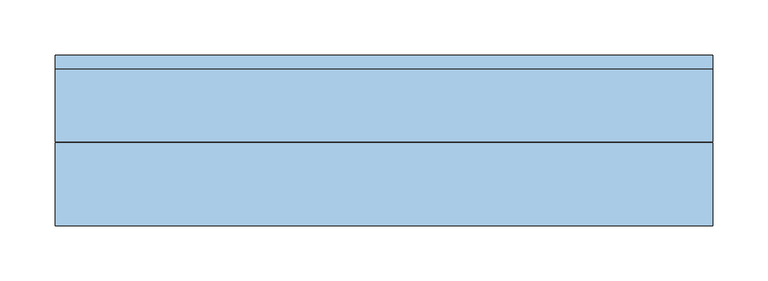
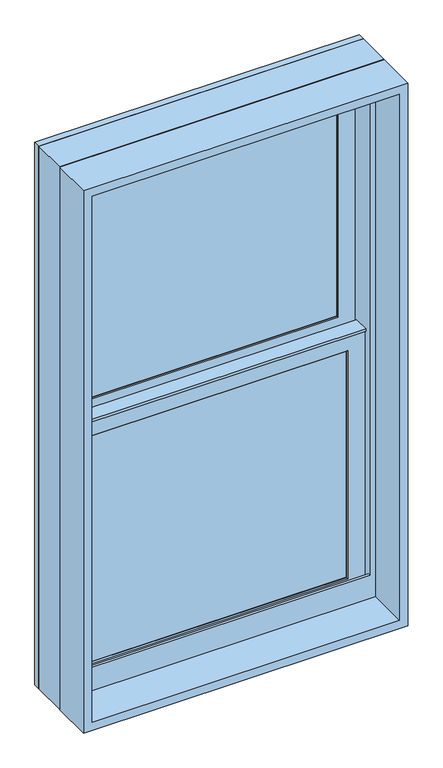
"""IFC4 building model written with IfcOpenShell, lengths in millimetres: window geometry, Window-Double_Hung-Marvin-Essential : ESDH2036."""

from ifc_helpers import new_model, si_unit, frame, origin, place, context, project, spatial, polyline, outline, extrude, faceted_brep, source, transform, mapped, element, save


def window_21fe58db(model_context):
    return source(origin(), model_context, "Body", "SolidModel", [
        extrude(outline(polyline([(89.9583333, 20.6375), (89.9583333, 15.875), (70.9083333, 15.875), (70.9083333, 20.6375), (89.9583333, 20.6375)])), frame((0.0, 0.0, 1441.45), z_axis=(0.0, 0.0, 1.0), x_axis=(1.0, 0.0, 0.0)), (0.0, 0.0, 1.0), 450.85),
        extrude(outline(polyline([(-70.9083333, 20.6375), (-70.9083333, 15.875), (-89.9583333, 15.875), (-89.9583333, 20.6375), (-70.9083333, 20.6375)])), frame((0.0, 0.0, 1441.45), z_axis=(0.0, 0.0, 1.0), x_axis=(1.0, 0.0, 0.0)), (0.0, 0.0, 1.0), 450.85),
        extrude(outline(polyline([(241.3, 20.6375), (241.3, 15.875), (-241.3, 15.875), (-241.3, 20.6375), (241.3, 20.6375)])), frame((0.0, 0.0, 1657.35), z_axis=(0.0, 0.0, 1.0), x_axis=(1.0, 0.0, 0.0)), (0.0, 0.0, 1.0), 19.05),
        extrude(outline(polyline([(-89.9583333, 46.83125), (-89.9583333, 51.59375), (-70.9083333, 51.59375), (-70.9083333, 46.83125), (-89.9583333, 46.83125)])), frame((0.0, 0.0, 1930.4), z_axis=(0.0, 0.0, 1.0), x_axis=(1.0, 0.0, 0.0)), (0.0, 0.0, 1.0), 450.85),
        extrude(outline(polyline([(70.9083333, 46.83125), (70.9083333, 51.59375), (89.9583333, 51.59375), (89.9583333, 46.83125), (70.9083333, 46.83125)])), frame((0.0, 0.0, 1930.4), z_axis=(0.0, 0.0, 1.0), x_axis=(1.0, 0.0, 0.0)), (0.0, 0.0, 1.0), 450.85),
        extrude(outline(polyline([(-241.3, 46.83125), (-241.3, 51.59375), (241.3, 51.59375), (241.3, 46.83125), (-241.3, 46.83125)])), frame((0.0, 0.0, 2146.3), z_axis=(0.0, 0.0, 1.0), x_axis=(1.0, 0.0, 0.0)), (0.0, 0.0, 1.0), 19.05),
        extrude(outline(polyline([(89.9583333, 20.6375), (70.9083333, 20.6375), (70.9083333, 25.4), (89.9583333, 25.4), (89.9583333, 20.6375)])), frame((0.0, 0.0, 1441.45), z_axis=(0.0, 0.0, 1.0), x_axis=(1.0, 0.0, 0.0)), (0.0, 0.0, 1.0), 450.85),
        extrude(outline(polyline([(-70.9083333, 20.6375), (-89.9583333, 20.6375), (-89.9583333, 25.4), (-70.9083333, 25.4), (-70.9083333, 20.6375)])), frame((0.0, 0.0, 1441.45), z_axis=(0.0, 0.0, 1.0), x_axis=(1.0, 0.0, 0.0)), (0.0, 0.0, 1.0), 450.85),
        extrude(outline(polyline([(241.3, 20.6375), (-241.3, 20.6375), (-241.3, 25.4), (241.3, 25.4), (241.3, 20.6375)])), frame((0.0, 0.0, 1657.35), z_axis=(0.0, 0.0, 1.0), x_axis=(1.0, 0.0, 0.0)), (0.0, 0.0, 1.0), 19.05),
        extrude(outline(polyline([(-89.9583333, 56.35625), (-70.9083333, 56.35625), (-70.9083333, 51.59375), (-89.9583333, 51.59375), (-89.9583333, 56.35625)])), frame((0.0, 0.0, 1930.4), z_axis=(0.0, 0.0, 1.0), x_axis=(1.0, 0.0, 0.0)), (0.0, 0.0, 1.0), 450.85),
        extrude(outline(polyline([(70.9083333, 56.35625), (89.9583333, 56.35625), (89.9583333, 51.59375), (70.9083333, 51.59375), (70.9083333, 56.35625)])), frame((0.0, 0.0, 1930.4), z_axis=(0.0, 0.0, 1.0), x_axis=(1.0, 0.0, 0.0)), (0.0, 0.0, 1.0), 450.85),
        extrude(outline(polyline([(-241.3, 56.35625), (241.3, 56.35625), (241.3, 51.59375), (-241.3, 51.59375), (-241.3, 56.35625)])), frame((0.0, 0.0, 2146.3), z_axis=(0.0, 0.0, 1.0), x_axis=(1.0, 0.0, 0.0)), (0.0, 0.0, 1.0), 19.05),
        faceted_brep([(-268.2875, 5.6780605, 1922.3351748), (-268.2875, 5.6780605, 1917.7), (268.2875, 5.6780605, 1917.7), (268.2875, 5.6780605, 1922.3351748), (-268.2875, 34.8118605, 1922.3351748), (268.2875, 34.8118605, 1922.3351748), (268.2875, 34.8118605, 1917.7), (-268.2875, 34.8118605, 1917.7), (-268.2875, 30.1625, 1917.7), (-268.2875, 30.1625, 1414.4625), (-268.2875, 8.9241104, 1414.4625), (-268.2875, 8.9241104, 1917.7), (268.2875, 8.9241104, 1917.7), (268.2875, 30.1625, 1917.7), (268.2875, 8.9241104, 1414.4625), (268.2875, 30.1625, 1414.4625), (-252.4034752, 11.90625, 1903.4034752), (-252.4034752, 30.1625, 1903.4034752), (252.4034752, 30.1625, 1903.4034752), (252.4034752, 11.90625, 1903.4034752), (-235.74375, 10.4662439, 1886.74375), (-235.74375, 11.90625, 1886.74375), (235.74375, 11.90625, 1886.74375), (235.74375, 10.4662439, 1886.74375), (237.2858834, 8.9241104, 1888.2858834), (-237.2858834, 8.9241104, 1888.2858834), (252.4034752, 30.1625, 1430.3465248), (252.4034752, 11.90625, 1430.3465248), (235.74375, 11.90625, 1447.00625), (235.74375, 10.4662439, 1447.00625), (237.2858834, 8.9241104, 1445.4641166), (-252.4034752, 30.1625, 1430.3465248), (-252.4034752, 11.90625, 1430.3465248), (-235.74375, 11.90625, 1447.00625), (-235.74375, 10.4662439, 1447.00625), (-237.2858834, 8.9241104, 1445.4641166)], [[[0, 1, 2, 3]], [[4, 5, 6, 7]], [[1, 0, 4, 7, 8, 9, 10, 11]], [[2, 1, 11, 12]], [[7, 6, 13, 8]], [[3, 2, 12, 14, 15, 13, 6, 5]], [[0, 3, 5, 4]], [[16, 17, 18, 19]], [[20, 21, 22, 23]], [[20, 23, 24, 25]], [[19, 18, 26, 27]], [[23, 22, 28, 29]], [[24, 23, 29, 30]], [[27, 26, 31, 32]], [[29, 28, 33, 34]], [[30, 29, 34, 35]], [[15, 14, 10, 9]], [[15, 9, 8, 13], [18, 17, 31, 26]], [[17, 16, 32, 31]], [[16, 19, 27, 32], [22, 21, 33, 28]], [[21, 20, 34, 33]], [[20, 25, 35, 34]], [[10, 14, 12, 11], [25, 24, 30, 35]]]),
        extrude(outline(polyline([(38.5955581, 1903.4125), (33.5778968, 1903.4125), (33.5778968, 1905.0), (39.9405976, 1905.0), (39.9405976, 1903.4125), (61.515625, 1903.4125), (47.6307501, 1900.0975159), (38.5955581, 1900.0975159), (38.5955581, 1903.4125)])), frame((-268.2875, 0.0, 0.0), z_axis=(1.0, 0.0, 0.0), x_axis=(0.0, 1.0, 0.0)), (0.0, 0.0, 1.0), 536.575),
        faceted_brep([(298.45, 0.0, 1384.3), (298.45, 0.0, 2438.4), (-298.45, 0.0, 2438.4), (-298.45, 0.0, 1384.3), (272.25625, 0.0, 1445.41875), (-272.25625, 0.0, 1445.41875), (-272.25625, 0.0, 2412.20625), (272.25625, 0.0, 2412.20625), (272.25625, 3.96875, 1384.3), (-272.25625, 3.96875, 1384.3), (-272.25625, 3.96875, 1445.41875), (272.25625, 3.96875, 1445.41875), (-298.45, 65.6828125, 1384.3), (-272.25625, 65.6828125, 1384.3), (272.25625, 65.6828125, 1384.3), (298.45, 65.6828125, 1384.3), (-298.45, 65.6828125, 2438.4), (298.45, 65.6828125, 2438.4), (272.25625, 65.6828125, 2412.20625), (-272.25625, 65.6828125, 2412.20625)], [[[0, 1, 2, 3], [4, 5, 6, 7]], [[8, 9, 10, 11]], [[5, 4, 11, 10]], [[0, 3, 12, 13, 9, 8, 14, 15]], [[13, 12, 16, 17, 15, 14, 18, 19]], [[13, 19, 6, 5, 10, 9]], [[7, 6, 19, 18]], [[18, 14, 8, 11, 4, 7]], [[1, 0, 15, 17]], [[2, 1, 17, 16]], [[3, 2, 16, 12]]]),
        faceted_brep([(272.25625, 30.1625, 1911.35), (270.66875, 30.1625, 1911.35), (270.66875, 30.1625, 1408.6544613), (272.25625, 30.1625, 1408.6544613), (-270.66875, 30.1625, 1911.35), (-272.25625, 30.1625, 1911.35), (-272.25625, 30.1625, 1408.6544613), (-270.66875, 30.1625, 1408.6544613), (270.66875, 63.5, 1911.35), (272.25625, 63.5, 1911.35), (272.25625, 63.5, 1402.1743077), (270.66875, 63.5, 1402.1743077), (-272.25625, 63.5, 1911.35), (-270.66875, 63.5, 1911.35), (-270.66875, 63.5, 1402.1743077), (-272.25625, 63.5, 1402.1743077), (283.5108932, 3.96875, 1413.7460105), (283.5108932, 3.96875, 1384.3), (283.5108932, 65.6828125, 1384.3), (283.5108932, 65.6828125, 1401.750012), (-283.5108932, 3.96875, 1384.3), (-283.5108932, 3.96875, 1413.7460105), (-283.5108932, 65.6828125, 1401.750012), (-283.5108932, 65.6828125, 1384.3), (283.5108932, 78.58125, 1399.2428097), (-283.5108932, 78.58125, 1399.2428097), (-281.4971252, 68.2348864, 1401.2539391), (-263.53135, 68.2348864, 1401.2539391), (-263.53135, 65.6828125, 1401.750012), (263.53135, 65.6828125, 1401.750012), (263.53135, 68.2348864, 1401.2539391), (281.4971252, 68.2348864, 1401.2539391), (-298.45, 65.6828125, 1384.3), (-298.45, 78.5948249, 1384.3), (298.45, 78.5948249, 1384.3), (298.45, 65.6828125, 1384.3), (-298.45, 78.58125, 2438.4), (298.45, 78.58125, 2438.4), (283.5108932, 78.58125, 2423.4608932), (-283.5108932, 78.58125, 2423.4608932), (-298.45, 65.6828125, 2438.4), (-281.4971252, 68.2348864, 2421.4471252), (281.4971252, 68.2348864, 2421.4471252), (263.53135, 68.2348864, 2403.48135), (-263.53135, 68.2348864, 2403.48135), (-263.53135, 65.6828125, 2403.48135), (263.53135, 65.6828125, 2403.48135), (298.45, 65.6828125, 2438.4)], [[[0, 1, 2, 3]], [[4, 5, 6, 7]], [[8, 9, 10, 11]], [[12, 13, 14, 15]], [[1, 8, 11, 2]], [[9, 0, 3, 10]], [[1, 0, 9, 8]], [[5, 4, 13, 12]], [[5, 12, 15, 6]], [[13, 4, 7, 14]], [[16, 17, 18, 19]], [[20, 21, 22, 23]], [[24, 25, 26, 27, 28, 22, 21, 16, 19, 29, 30, 31], [3, 2, 11, 10], [7, 6, 15, 14]], [[17, 16, 21, 20]], [[17, 20, 23, 32, 33, 34, 35, 18]], [[34, 33, 36, 37], [25, 24, 38, 39]], [[33, 32, 40, 36]], [[39, 41, 26, 25]], [[41, 42, 31, 30, 43, 44, 27, 26]], [[44, 45, 28, 27]], [[40, 32, 23, 22, 28, 45, 46, 29, 19, 18, 35, 47]], [[36, 40, 47, 37]], [[39, 38, 42, 41]], [[44, 43, 46, 45]], [[34, 37, 47, 35]], [[42, 38, 24, 31]], [[46, 43, 30, 29]]]),
        extrude(outline(polyline([(248.44375, 11.90625), (-248.44375, 11.90625), (-248.44375, 15.08125), (248.44375, 15.08125), (248.44375, 11.90625)])), frame((0.0, 0.0, 1434.30625), z_axis=(0.0, 0.0, 1.0), x_axis=(1.0, 0.0, 0.0)), (0.0, 0.0, 1.0), 465.1375),
        extrude(outline(polyline([(248.44375, 42.8625), (-248.44375, 42.8625), (-248.44375, 46.0375), (248.44375, 46.0375), (248.44375, 42.8625)])), frame((0.0, 0.0, 1923.25625), z_axis=(0.0, 0.0, 1.0), x_axis=(1.0, 0.0, 0.0)), (0.0, 0.0, 1.0), 465.1375),
        faceted_brep([(-235.74375, 31.194477, 1886.74375), (-237.2858834, 32.7366104, 1888.2858834), (237.2858834, 32.7366104, 1888.2858834), (235.74375, 31.194477, 1886.74375), (-235.74375, 30.1625, 1886.74375), (235.74375, 30.1625, 1886.74375), (-268.2875, 32.7366104, 1919.2875), (-268.2875, 30.1625, 1919.2875), (268.2875, 30.1625, 1919.2875), (268.2875, 32.7366104, 1919.2875), (237.2858834, 32.7366104, 1445.4641166), (235.74375, 31.194477, 1447.00625), (235.74375, 30.1625, 1447.00625), (268.2875, 30.1625, 1414.4625), (268.2875, 32.7366104, 1414.4625), (-237.2858834, 32.7366104, 1445.4641166), (-235.74375, 31.194477, 1447.00625), (-235.74375, 30.1625, 1447.00625), (-268.2875, 30.1625, 1414.4625), (-268.2875, 32.7366104, 1414.4625)], [[[0, 1, 2, 3]], [[4, 0, 3, 5]], [[6, 7, 8, 9]], [[3, 2, 10, 11]], [[5, 3, 11, 12]], [[9, 8, 13, 14]], [[11, 10, 15, 16]], [[12, 11, 16, 17]], [[14, 13, 18, 19]], [[9, 14, 19, 6], [1, 15, 10, 2]], [[16, 15, 1, 0]], [[17, 16, 0, 4]], [[7, 18, 13, 8], [5, 12, 17, 4]], [[19, 18, 7, 6]]]),
        faceted_brep([(-252.4034752, 42.8625, 2392.3534752), (-252.4034752, 61.11875, 2392.3534752), (252.4034752, 61.11875, 2392.3534752), (252.4034752, 42.8625, 2392.3534752), (-235.74375, 41.4224939, 2375.69375), (-235.74375, 42.8625, 2375.69375), (235.74375, 42.8625, 2375.69375), (235.74375, 41.4224939, 2375.69375), (-237.2858834, 39.8803604, 2377.2358834), (237.2858834, 39.8803604, 2377.2358834), (-268.2875, 61.11875, 2408.2375), (-268.2875, 39.8803604, 2408.2375), (268.2875, 39.8803604, 2408.2375), (268.2875, 61.11875, 2408.2375), (252.4034752, 61.11875, 1919.2965248), (252.4034752, 42.8625, 1919.2965248), (235.74375, 42.8625, 1935.95625), (235.74375, 41.4224939, 1935.95625), (237.2858834, 39.8803604, 1934.4141166), (268.2875, 39.8803604, 1903.4125), (268.2875, 61.11875, 1903.4125), (-252.4034752, 61.11875, 1919.2965248), (-252.4034752, 42.8625, 1919.2965248), (-235.74375, 42.8625, 1935.95625), (-235.74375, 41.4224939, 1935.95625), (-237.2858834, 39.8803604, 1934.4141166), (-268.2875, 39.8803604, 1903.4125), (-268.2875, 61.11875, 1903.4125)], [[[0, 1, 2, 3]], [[4, 5, 6, 7]], [[8, 4, 7, 9]], [[10, 11, 12, 13]], [[3, 2, 14, 15]], [[7, 6, 16, 17]], [[9, 7, 17, 18]], [[13, 12, 19, 20]], [[15, 14, 21, 22]], [[17, 16, 23, 24]], [[18, 17, 24, 25]], [[20, 19, 26, 27]], [[13, 20, 27, 10], [1, 21, 14, 2]], [[22, 21, 1, 0]], [[3, 15, 22, 0], [5, 23, 16, 6]], [[24, 23, 5, 4]], [[25, 24, 4, 8]], [[11, 26, 19, 12], [9, 18, 25, 8]], [[27, 26, 11, 10]]]),
        faceted_brep([(-268.2875, 61.11875, 1903.4125), (-268.2875, 63.6928604, 1903.4125), (268.2875, 63.6928604, 1903.4125), (268.2875, 61.11875, 1903.4125), (-235.74375, 62.150727, 1935.95625), (-235.74375, 61.11875, 1935.95625), (235.74375, 61.11875, 1935.95625), (235.74375, 62.150727, 1935.95625), (-237.2858834, 63.6928604, 1934.4141166), (237.2858834, 63.6928604, 1934.4141166), (268.2875, 63.6928604, 2408.2375), (268.2875, 61.11875, 2408.2375), (235.74375, 61.11875, 2375.69375), (235.74375, 62.150727, 2375.69375), (237.2858834, 63.6928604, 2377.2358834), (-268.2875, 63.6928604, 2408.2375), (-268.2875, 61.11875, 2408.2375), (-235.74375, 61.11875, 2375.69375), (-235.74375, 62.150727, 2375.69375), (-237.2858834, 63.6928604, 2377.2358834)], [[[0, 1, 2, 3]], [[4, 5, 6, 7]], [[8, 4, 7, 9]], [[3, 2, 10, 11]], [[7, 6, 12, 13]], [[9, 7, 13, 14]], [[11, 10, 15, 16]], [[13, 12, 17, 18]], [[14, 13, 18, 19]], [[16, 15, 1, 0]], [[3, 11, 16, 0], [5, 17, 12, 6]], [[18, 17, 5, 4]], [[19, 18, 4, 8]], [[1, 15, 10, 2], [9, 14, 19, 8]]]),
        extrude(outline(polyline([(248.44375, 26.19375), (-248.44375, 26.19375), (-248.44375, 30.1625), (248.44375, 30.1625), (248.44375, 26.19375)])), frame((0.0, 0.0, 1434.30625), z_axis=(0.0, 0.0, 1.0), x_axis=(1.0, 0.0, 0.0)), (0.0, 0.0, 1.0), 465.1375),
        extrude(outline(polyline([(248.44375, 57.15), (-248.44375, 57.15), (-248.44375, 61.11875), (248.44375, 61.11875), (248.44375, 57.15)])), frame((0.0, 0.0, 1923.25625), z_axis=(0.0, 0.0, 1.0), x_axis=(1.0, 0.0, 0.0)), (0.0, 0.0, 1.0), 465.1375),
        extrude(outline(polyline([(2438.4, 298.45), (2438.4, -298.45), (1384.3, -298.45), (1384.3, 298.45), (2438.4, 298.45)]), holes=[polyline([(2422.525, 282.575), (1400.175, 282.575), (1400.175, -282.575), (2422.525, -282.575), (2422.525, 282.575)])]), frame((0.0, -76.2, 0.0), z_axis=(0.0, 1.0, 0.0), x_axis=(0.0, 0.0, 1.0)), (0.0, 0.0, 1.0), 75.40625),
    ])


if __name__ == "__main__":
    model = new_model("IFC4")
    model_context = context("Model", 3, world=origin())
    ifc_project = project(units=[si_unit("LENGTHUNIT", "METRE", prefix="MILLI")], contexts=[model_context])
    site = spatial("IfcSite", under=ifc_project)
    building = spatial("IfcBuilding", under=site)
    placement = place(None, origin())
    window_shape = window_21fe58db(model_context)
    element("IfcWindow", 1, ObjectType="Window-Double_Hung-Marvin-Essential : ESDH2036", at=placement, inside=building, context=model_context, shape_type="MappedRepresentation", body=[
        mapped(window_shape, transform((0.0, 0.0, 0.0), x_axis=(1.0, 0.0, 0.0), y_axis=(0.0, 1.0, 0.0), z_axis=(0.0, 0.0, 1.0))),
    ])
    save(model, "model.ifc")

# Revit data of these elements
# Type "Window-Double_Hung-Marvin-Essential : ESDH2036"
#   Type Mark = "41"
#   Window Type = "Essential Double Hung"
#   Product data url = "https://bimobject.com/marvin-windows-and-doors/product/marvin-dhwau"
#   Product Guid = "c4a96547-874c-4385-91dc-a058adc19d98"
#   Frame = "All Ultrex"
#   Egress Window = "No"
#   URL = "www.marvin.com"
#   Model = "ESDH2036"
#   Manufacturer = "Marvin Windows and Doors"
#   Label Egress = ""
#   Glass Type = "IG Low E II with Argon"
#   Design Pressure = "DP50"
#   Description = "2442 DBHG"
#   Analytic Construction = "<None>"
#   Prairie Corner Width = 0' - 4"
#   Prairie Corner Height = 0' - 4"
#   Egress Width = 1' - 8 9/16"
#   Egress Height = 1' - 4 27/128"
#   Rough Width = 2' - 0"
#   Rough Height = 3' - 6"
#   Nominal Width = 2' - 0"
#   Nominal Height = 3' - 6"
#   Inset to Installation Flange [instance default] = 0' - 1"
#   Height = 3' - 5 1/2"
#   Egress Area = 2.31484 SF
#   Default Head Height = 8' - 0"
#   Width = 1' - 11 1/2"
#   Daylight Area = 4.46338 SF
#   DLO Width = 1' - 6 9/16"
#   DLO Height = 1' - 5 5/16"
#   Muntins Top Sash = yes
#   Lites Wide Top Sash = 3
#   Lites Wide Bottom Sash = 3
#   Lites High Top Sash = 2
#   Lites High Bottom Sash = 2
#   Lite Cut Prairie 9 = no
#   Lite Cut HV Grid = yes
#   Muntins Bottom Sash = yes
#   Label Visibility = no
#   Jamb Extension Visibility = yes
#   Edition number = 1
#   Interior Material = Ultrex-Marvin-Stonewhite
#   Glazing Material = Glass-Marvin-IG Low E II with Argon
#   Cladding Material = Ultrex-Marvin-Pebblegray
#   Wall Closure = (empty or 0)
#   Assembly Code = ""
# Element 1 (IfcWindow, "Window-Double_Hung-Marvin-Essential : ESDH2036")
#   Materials on its faces: "Ultrex-Marvin-Pebblegray", "Ultrex-Marvin-Stonewhite", "Glass-Marvin-IG Low E II with Argon"
# Materials
#   "Ultrex-Marvin-Stonewhite": class "Paint", colour RGB 250 251 245, transparency 0
#   "Glass-Marvin-IG Low E II with Argon": class "Glass", colour RGB 0 128 192, transparency 0.85
#   "Ultrex-Marvin-Pebblegray": class "Paint", colour RGB 189 185 173, transparency 0
